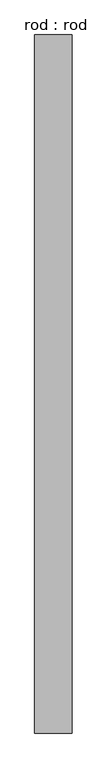
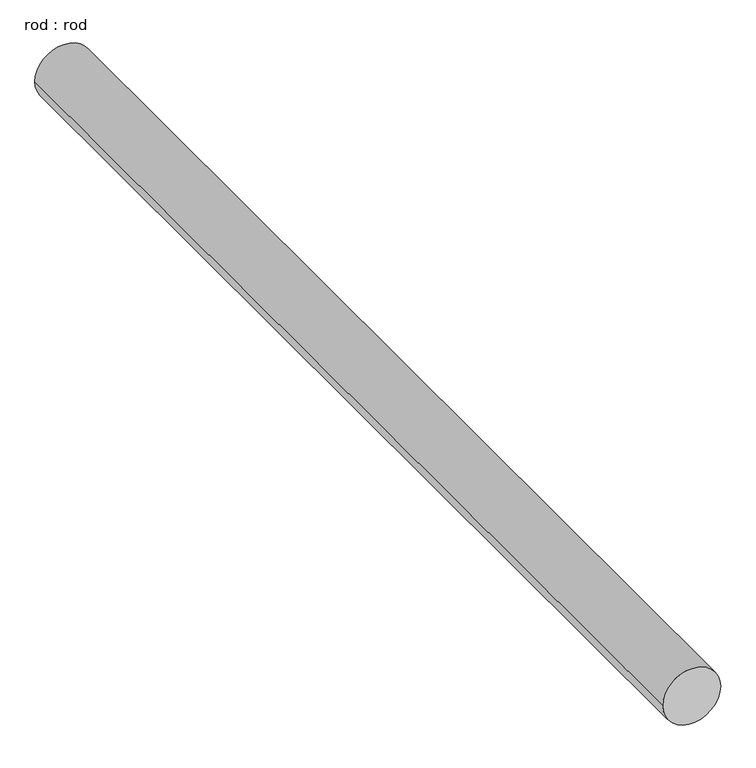
"""IFC4 building model written with IfcOpenShell, lengths in millimetres: proxy geometry, rod : rod."""

from ifc_helpers import new_model, si_unit, point, frame, frame_2d, origin, place, context, project, spatial, circle_curve, trimmed, segment, composite_curve, outline, extrude, source, transform, mapped, element, save


def rod_rod_3924ccb1(model_context):
    return source(origin(), model_context, "Body", "SweptSolid", [
        extrude(outline(composite_curve([segment(trimmed(circle_curve(frame_2d((0.0108462, 0.0)), 200.0), [point((0.0108462, 200.0))], [point((0.0108462, -200.0))], False, "CARTESIAN"), True, "CONTINUOUS"), segment(trimmed(circle_curve(frame_2d((0.0108462, 0.0)), 200.0), [point((0.0108462, -200.0))], [point((0.0108462, 200.0))], False, "CARTESIAN"), True, "CONTINUOUS")], self_intersect=False)), frame((0.0, 347.5650675, 0.0), z_axis=(0.0, 1.0, 0.0), x_axis=(0.0, 0.0, 1.0)), (0.0, 0.0, 1.0), 7490.3270957),
    ])


if __name__ == "__main__":
    model = new_model("IFC4")
    model_context = context("Model", 3, world=origin())
    ifc_project = project(units=[si_unit("LENGTHUNIT", "METRE", prefix="MILLI")], contexts=[model_context])
    site = spatial("IfcSite", under=ifc_project)
    building = spatial("IfcBuilding", under=site)
    placement = place(None, origin())
    rod_rod_shape = rod_rod_3924ccb1(model_context)
    element("IfcBuildingElementProxy", 1, Name="rod : rod", ObjectType="rod : rod", at=placement, inside=building, context=model_context, shape_type="MappedRepresentation", body=[
        mapped(rod_rod_shape, transform((0.0, 0.0, 0.0), x_axis=(1.0, 0.0, 0.0), y_axis=(0.0, 1.0, 0.0), z_axis=(0.0, 0.0, 1.0))),
    ])
    save(model, "model.ifc")

# Revit data of these elements
# Type "rod : rod"
#   Default Elevation = 0
